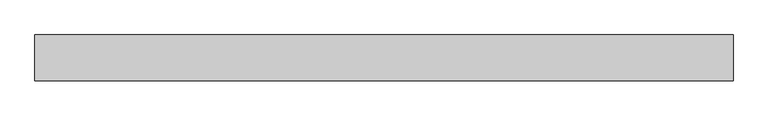
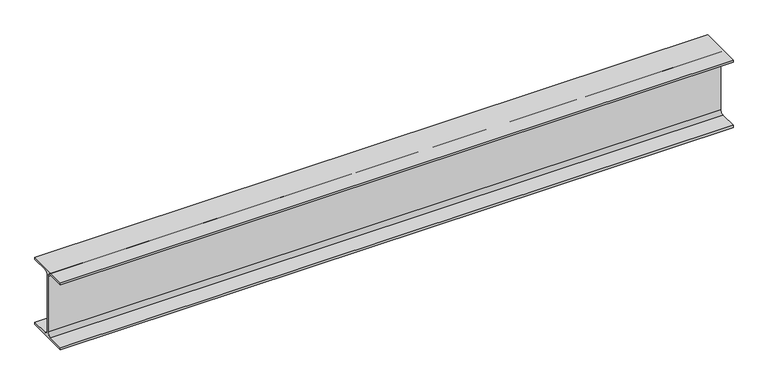
"""IFC4 building model written with IfcOpenShell, lengths in millimetres: beam geometry, 0912_Steel Framing_H-KSD3502 : H_SB_ASB_H-482x300x11x15."""

from ifc_helpers import new_model, si_unit, point, frame, frame_2d, origin, place, context, project, spatial, polyline, circle_curve, trimmed, segment, composite_curve, outline, extrude, source, transform, mapped, element, save


def beam_69ae5304(model_context):
    return source(origin(), model_context, "Body", "SweptSolid", [
        extrude(outline(composite_curve([segment(polyline([(150.0, -226.0), (150.0, -241.0), (-150.0, -241.0), (-150.0, -226.0), (-31.5, -226.0)]), True, "CONTINUOUS"), segment(trimmed(circle_curve(frame_2d((-31.5, -200.0)), 26.0), [point((-31.5, -226.0))], [point((-5.5, -200.0))], True, "CARTESIAN"), True, "CONTINUOUS"), segment(polyline([(-5.5, -200.0), (-5.5, 200.0)]), True, "CONTINUOUS"), segment(trimmed(circle_curve(frame_2d((-31.5, 200.0)), 26.0), [point((-5.5, 200.0))], [point((-31.5, 226.0))], True, "CARTESIAN"), True, "CONTINUOUS"), segment(polyline([(-31.5, 226.0), (-150.0, 226.0), (-150.0, 241.0), (150.0, 241.0), (150.0, 226.0), (31.5, 226.0)]), True, "CONTINUOUS"), segment(trimmed(circle_curve(frame_2d((31.5, 200.0)), 26.0), [point((31.5, 226.0))], [point((5.5, 200.0))], True, "CARTESIAN"), True, "CONTINUOUS"), segment(polyline([(5.5, 200.0), (5.5, -200.0)]), True, "CONTINUOUS"), segment(trimmed(circle_curve(frame_2d((31.5, -200.0)), 26.0), [point((5.5, -200.0))], [point((31.5, -226.0))], True, "CARTESIAN"), True, "CONTINUOUS"), segment(polyline([(31.5, -226.0), (150.0, -226.0)]), True, "CONTINUOUS")], self_intersect=False)), frame((-2279.8, 0.0, 0.0), z_axis=(1.0, 0.0, 0.0), x_axis=(0.0, 1.0, 0.0)), (0.0, 0.0, 1.0), 4559.6),
    ])


if __name__ == "__main__":
    model = new_model("IFC4")
    model_context = context("Model", 3, world=origin())
    ifc_project = project(units=[si_unit("LENGTHUNIT", "METRE", prefix="MILLI")], contexts=[model_context])
    site = spatial("IfcSite", under=ifc_project)
    building = spatial("IfcBuilding", under=site)
    placement = place(None, origin())
    beam_shape = beam_69ae5304(model_context)
    element("IfcBeam", 1, ObjectType="0912_Steel Framing_H-KSD3502 : H_SB_ASB_H-482x300x11x15", at=placement, inside=building, context=model_context, shape_type="MappedRepresentation", body=[
        mapped(beam_shape, transform((0.0, 0.0, 0.0), x_axis=(1.0, 0.0, 0.0), y_axis=(0.0, 1.0, 0.0), z_axis=(0.0, 0.0, 1.0))),
    ])
    save(model, "model.ifc")

# Revit data of these elements
# Type "0912_Steel Framing_H-KSD3502 : H_SB_ASB_H-482x300x11x15"
#   H_WM Code_1 = "S01AA001-00001 | Main Steel Structure Fabrication Work | Shelter/Building | Heavy Steel - Standard (Weight≥90KG/M) | Material: (   )"
#   H_WM Code_2 = "S03AA027-00001 | Main Steel Structure Erection Work | Shelter/Building | Heavy Steel (Weight≥90KG/M) | Material: (   )"
#   H_WM Code_3 = "S01AA010-00001 | Main Steel Structure Fabrication Work | Shelter/Building | Steel Painting/Coating | for Non-Fireproofed Steel Surface, Surface Preparation, Primer, Second & Final Coat | Material: (   )"
#   H_Q'ty Cal Type Tag = "SB-Q2"
#   Width = 30.0 cm
#   Web Thickness = 1.1 cm
#   Web Fillet = 2.6 cm
#   Warping Constant = 3680000.0 cm⁶
#   W = 0
#   Torsional Moment of Inertia = 88.2192 cm⁴
#   Section Area = 145.5 cm²
#   Plastic Modulus weak axis = 695.0 cm³
#   Plastic Modulus strong axis = 2790.0 cm³
#   Perimeter = 2.10 m²/m
#   Nominal Weight = 114.00 kgf/m
#   Moment of Inertia weak axis = 6760.00 cm⁴
#   Moment of Inertia strong axis = 60400.00 cm⁴
#   Height = 48.2 cm
#   Flange Thickness = 1.5 cm
#   Elastic Modulus weak axis = 451.0 cm³
#   Elastic Modulus strong axis = 2500.0 cm³
#   Centroid Vertical = 24.1 cm
#   Centroid Horizontal = 15.0 cm
#   Ix = 604000000
#   Length [instance default] = 1.5240 m
#   Zx = 2790000
#   b = 0.3000 m
#   h = 0.4820 m
#   r = 0.0260 m
#   s = 0.0110 m
#   t = 0.0150 m
#   A = 0.01455 m²
#   Structural Material [instance default] = Steel, 45-345
#   Assembly Code = ""
# Element 1 (IfcBeam, "0912_Steel Framing_H-KSD3502 : H_SB_ASB_H-482x300x11x15")
#   Structural Material = none
# Materials
#   "Steel, 45-345": class "Metal", colour RGB 189 187 185, transparency 0, Description = "Steel 345 MPa", Cost = 0
